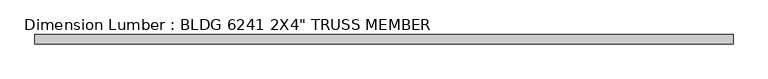
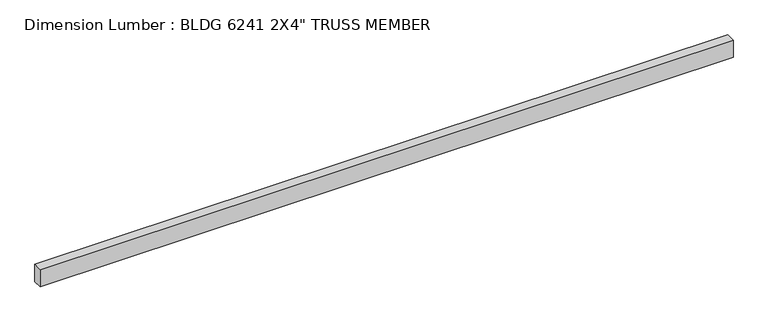
"""IFC4 building model written with IfcOpenShell, lengths in millimetres: beam geometry."""

from ifc_helpers import new_model, si_unit, frame, origin, place, context, project, spatial, polyline, outline, extrude, source, transform, mapped, element, save


def beam_32b3ca21(model_context):
    return source(origin(), model_context, "Body", "SweptSolid", [
        extrude(outline(polyline([(1914.525, 25.4), (1914.525, -25.4), (-1939.925, -25.4), (-1939.925, 25.4), (1914.525, 25.4)])), frame((0.0, 0.0, -50.8), z_axis=(0.0, 0.0, 1.0), x_axis=(1.0, 0.0, 0.0)), (0.0, 0.0, 1.0), 101.6),
    ])


if __name__ == "__main__":
    model = new_model("IFC4")
    model_context = context("Model", 3, world=origin())
    ifc_project = project(units=[si_unit("LENGTHUNIT", "METRE", prefix="MILLI")], contexts=[model_context])
    site = spatial("IfcSite", under=ifc_project)
    building = spatial("IfcBuilding", under=site)
    placement = place(None, origin())
    beam_shape = beam_32b3ca21(model_context)
    element("IfcBeam", 1, ObjectType="Dimension Lumber : BLDG 6241 2X4\" TRUSS MEMBER", at=placement, inside=building, context=model_context, shape_type="MappedRepresentation", body=[
        mapped(beam_shape, transform((0.0, 0.0, 0.0), x_axis=(1.0, 0.0, 0.0), y_axis=(0.0, 1.0, 0.0), z_axis=(0.0, 0.0, 1.0))),
    ])
    save(model, "model.ifc")

# Revit data of these elements
# Type "Dimension Lumber : BLDG 6241 2X4\" TRUSS MEMBER"
#   Assembly Code = "B10"
#   A = 0.273472 SF
#   Length [instance default] = 5' - 0"
#   b = 0' - 2"
#   d = 0' - 4"
#   Structural Material [instance default] = Softwood, Lumber
# Element 1 (IfcBeam, "Dimension Lumber : BLDG 6241 2X4\" TRUSS MEMBER")
#   Materials on its faces: "Softwood, Lumber"
# Materials
#   "Softwood, Lumber": class "Wood", colour RGB 223 192 134, transparency 0, Description = "Pinus Echinata", Cost = 0
